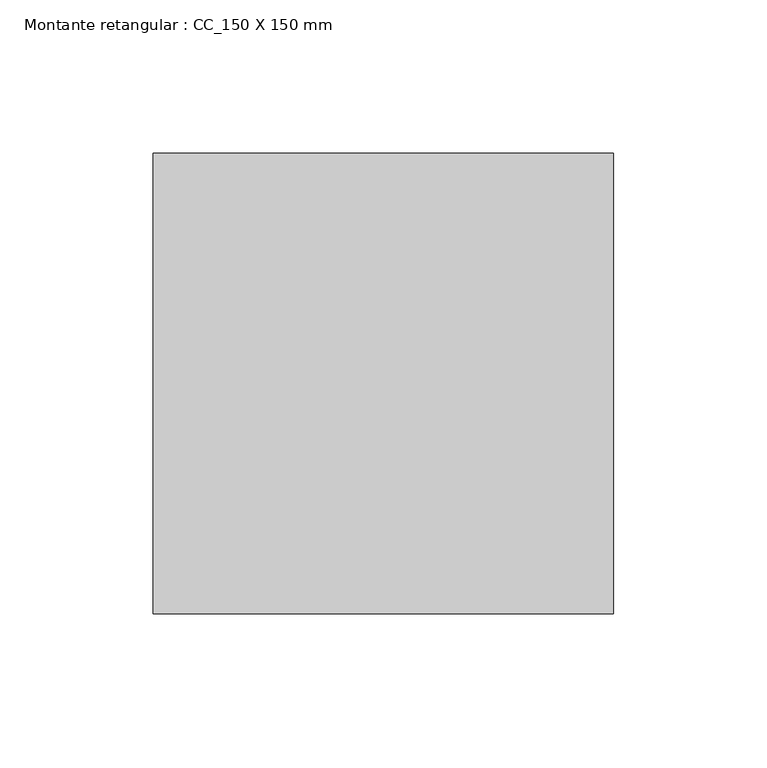
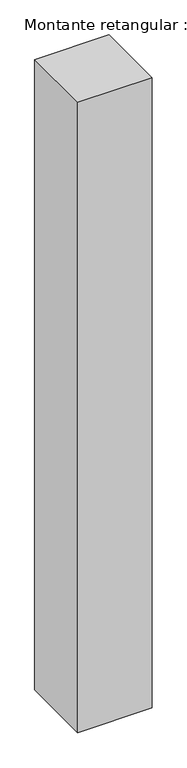
"""IFC4 building model written with IfcOpenShell, lengths in millimetres: member geometry, Montante retangular : CC_150 X 150 mm."""

from ifc_helpers import new_model, si_unit, frame, origin, place, context, project, spatial, polyline, outline, extrude, source, transform, mapped, element, save


def montante_retangular_cc_150_x_150_mm_106b3bff(model_context):
    return source(origin(), model_context, "Body", "SweptSolid", [
        extrude(outline(polyline([(0.0, 75.0), (0.0, -75.0), (-150.0, -75.0), (-150.0, 75.0), (0.0, 75.0)])), frame((0.0, 0.0, -1343.7500002), z_axis=(0.0, 0.0, 1.0), x_axis=(1.0, 0.0, 0.0)), (0.0, 0.0, 1.0), 1343.7500002),
    ])


if __name__ == "__main__":
    model = new_model("IFC4")
    model_context = context("Model", 3, world=origin())
    ifc_project = project(units=[si_unit("LENGTHUNIT", "METRE", prefix="MILLI")], contexts=[model_context])
    site = spatial("IfcSite", under=ifc_project)
    building = spatial("IfcBuilding", under=site)
    placement = place(None, origin())
    montante_retangular_cc_150_x_150_mm_shape = montante_retangular_cc_150_x_150_mm_106b3bff(model_context)
    element("IfcMember", 1, ObjectType="Montante retangular : CC_150 X 150 mm", at=placement, inside=building, context=model_context, shape_type="MappedRepresentation", body=[
        mapped(montante_retangular_cc_150_x_150_mm_shape, transform((0.0, 0.0, 0.0), x_axis=(1.0, 0.0, 0.0), y_axis=(0.0, 1.0, 0.0), z_axis=(0.0, 0.0, 1.0))),
    ])
    save(model, "model.ifc")

# Revit data of these elements
# Type "Montante retangular : CC_150 X 150 mm"
#   built-in parameter 1007304 = 0.492126 (stored number, unit not read)
#   built-in parameter 1007301 = 0.246063 (stored number, unit not read)
#   built-in parameter 1007300 = 0.246063 (stored number, unit not read)
# Element 1 (IfcMember, "Montante retangular : CC_150 X 150 mm")
#   Materials on its faces: ".ALUMÍNIO"
# Materials
#   ".ALUMÍNIO": class "CC_METAIS", colour RGB 244 244 244, transparency 0, Description = "Material alumínio", Cost = 0
